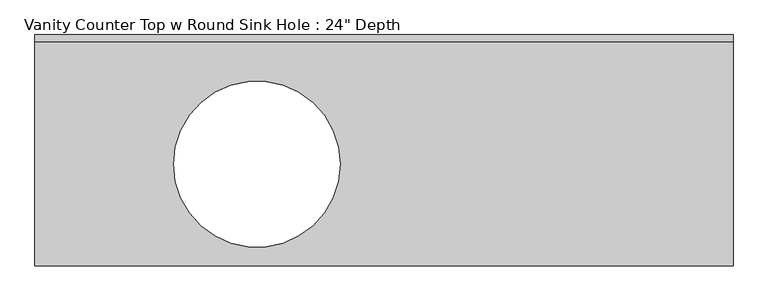
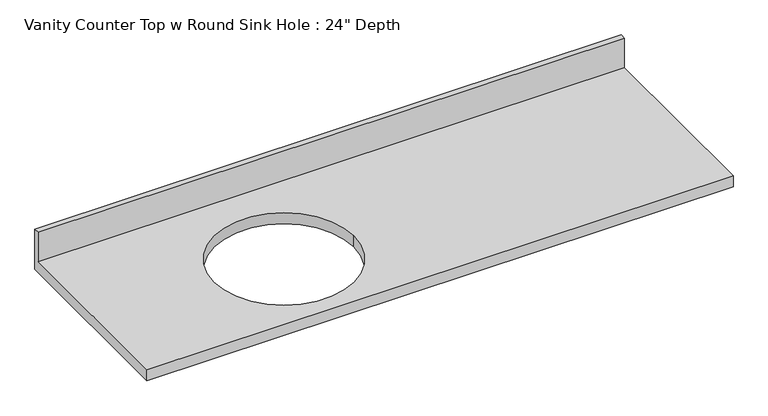
"""IFC4 building model written with IfcOpenShell, lengths in millimetres: furniture geometry."""

import ifcopenshell
import ifcopenshell.guid

model = None  # the IFC model being written
_history = None  # IfcOwnerHistory: only IFC2X3 demands one
_inside = {}  # id of a spatial element -> (the spatial element, [elements in it])
_under = {}  # id of a project, library or spatial element -> (it, [spatial elements below it])
_declared = {}  # id of a project -> (the project, [libraries it declares])
_typed = {}  # id of a type object -> (the type object, [elements of that type])
_made_of = {}  # id of a material, layer set ... -> (it, [elements and type objects made of it])


def new_model(schema):
    """Start an empty IFC model of exactly this schema.

    Asked for "IFC4X3", IfcOpenShell would pick the latest addendum, in which some entities
    have other attributes; the version numbers below select the first issue.
    IFC2X3 requires an IfcOwnerHistory on every rooted entity: one is made here for all.
    """
    global model, _history
    if schema == "IFC4X3":
        model = ifcopenshell.file(schema_version=(4, 3, 0, 0))
    else:
        model = ifcopenshell.file(schema=schema)
    _inside.clear()
    _under.clear()
    _declared.clear()
    _typed.clear()
    _made_of.clear()
    _history = None
    if model.schema == "IFC2X3":
        org = make("IfcOrganization", Name="unknown")
        user = make(
            "IfcPersonAndOrganization",
            ThePerson=make("IfcPerson", FamilyName="unknown"),
            TheOrganization=org,
        )
        app = make(
            "IfcApplication",
            ApplicationDeveloper=org,
            Version="unknown",
            ApplicationFullName="unknown",
            ApplicationIdentifier="unknown",
        )
        _history = make(
            "IfcOwnerHistory",
            OwningUser=user,
            OwningApplication=app,
            ChangeAction="ADDED",
            CreationDate=0,
        )
    return model


def make(cls, **values):
    """One entity of the class cls with the attributes given. An attribute that is None is left unset."""
    return model.create_entity(
        cls, **{name: value for name, value in values.items() if value is not None}
    )


def rooted(cls, **values):
    """An entity with a GlobalId (a new one), such as an element, a storey or a relation."""
    return make(cls, GlobalId=ifcopenshell.guid.new(), OwnerHistory=_history, **values)


def si_unit(unit_type, name, prefix=None):
    """IfcSIUnit, for example si_unit("LENGTHUNIT", "METRE", prefix="MILLI")."""
    return make("IfcSIUnit", UnitType=unit_type, Prefix=prefix, Name=name)


def assignment(units):
    """IfcUnitAssignment: the units of a project."""
    return None if units is None else make("IfcUnitAssignment", Units=units)


def point(xyz):
    """IfcCartesianPoint."""
    return None if xyz is None else make("IfcCartesianPoint", Coordinates=xyz)


def direction(xyz):
    """IfcDirection."""
    return None if xyz is None else make("IfcDirection", DirectionRatios=xyz)


def frame(location, z_axis=None, x_axis=None):
    """IfcAxis2Placement3D, a coordinate frame: its origin and axes. An axis left out is left unset."""
    return make(
        "IfcAxis2Placement3D",
        Location=point(location),
        Axis=direction(z_axis),
        RefDirection=direction(x_axis),
    )


def origin():
    """The frame at (0, 0, 0) with its axes left unset."""
    return frame((0.0, 0.0, 0.0))


def place(relative_to, where):
    """IfcLocalPlacement: puts the frame where relative to a parent placement (None: the world)."""
    return make(
        "IfcLocalPlacement", PlacementRelTo=relative_to, RelativePlacement=where
    )


def context(
    kind, dimensions, precision=None, world=None, true_north=None, identifier=None
):
    """IfcGeometricRepresentationContext, for example the 3D "Model" context."""
    return make(
        "IfcGeometricRepresentationContext",
        ContextIdentifier=identifier,
        ContextType=kind,
        CoordinateSpaceDimension=dimensions,
        Precision=precision,
        WorldCoordinateSystem=world,
        TrueNorth=true_north,
    )


def project(units=None, contexts=None):
    """IfcProject with its units and contexts."""
    return rooted(
        "IfcProject",
        Name="project",
        RepresentationContexts=contexts,
        UnitsInContext=assignment(units),
    )


def spatial(cls, under=None, at=None, **own):
    """A site, building, storey or space (cls), placed at a placement, below another one or the project."""
    s = rooted(cls, ObjectPlacement=at, **own)
    if under is not None:
        _under.setdefault(under.id(), (under, []))[1].append(s)
    return s


def polyline(points):
    """IfcPolyline through the points."""
    return make("IfcPolyline", Points=[point(p) for p in points])


def circle_curve(where, radius):
    """IfcCircle in the frame where."""
    return make("IfcCircle", Position=where, Radius=radius)


def shape(context_of_items, identifier, shape_type, items):
    """IfcShapeRepresentation: the items that make up one representation, for example the "Body"."""
    return make(
        "IfcShapeRepresentation",
        ContextOfItems=context_of_items,
        RepresentationIdentifier=identifier,
        RepresentationType=shape_type,
        Items=items,
    )


def source(mapping_origin, context_of_items, identifier, shape_type, items):
    """IfcRepresentationMap: a shape defined once, which mapped items show again and again."""
    return make(
        "IfcRepresentationMap",
        MappingOrigin=mapping_origin,
        MappedRepresentation=shape(context_of_items, identifier, shape_type, items),
    )


def transform(
    local_origin,
    x_axis=None,
    y_axis=None,
    z_axis=None,
    scale=None,
    scale2=None,
    scale3=None,
    uniform=True,
):
    """IfcCartesianTransformationOperator3D, or its non-uniform kind. x_axis, y_axis, z_axis: its Axis1, 2, 3."""
    if uniform:
        return make(
            "IfcCartesianTransformationOperator3D",
            Axis1=direction(x_axis),
            Axis2=direction(y_axis),
            LocalOrigin=point(local_origin),
            Scale=scale,
            Axis3=direction(z_axis),
        )
    return make(
        "IfcCartesianTransformationOperator3DnonUniform",
        Axis1=direction(x_axis),
        Axis2=direction(y_axis),
        LocalOrigin=point(local_origin),
        Scale=scale,
        Axis3=direction(z_axis),
        Scale2=scale2,
        Scale3=scale3,
    )


def mapped(mapping_source, mapping_target):
    """IfcMappedItem: shows the shape of a source again, moved by a transform."""
    return make(
        "IfcMappedItem", MappingSource=mapping_source, MappingTarget=mapping_target
    )


def made_of(thing, what):
    """Note that an element or type object is made of a material, layer set ...; save() writes the relation."""
    if what is not None:
        _made_of.setdefault(what.id(), (what, []))[1].append(thing)
    return thing


def element(
    cls,
    number,
    at=None,
    inside=None,
    cuts=None,
    type_object=None,
    material=None,
    context=None,
    identifier="Body",
    shape_type=None,
    held_by="IfcProductDefinitionShape",
    body=None,
    shapes=None,
    **own,
):
    """One element of the class cls, such as IfcWall. Its Tag is "e" and its number.

    at: its placement. inside: the storey or other place that contains it. cuts: it is an
    opening in that element (IfcRelVoidsElement). A single representation is given by context,
    identifier, shape_type and body (its items); several are given by shapes. held_by: the class
    of the entity that holds the representations. save() writes the other relations.
    """
    e = rooted(cls, Tag="e%d" % number, ObjectPlacement=at, **own)
    if body is not None:
        shapes = [shape(context, identifier, shape_type, body)]
    if shapes is not None:
        e.Representation = make(held_by, Representations=shapes)
    if inside is not None:
        _inside.setdefault(inside.id(), (inside, []))[1].append(e)
    if cuts is not None:
        rooted(
            "IfcRelVoidsElement", RelatingBuildingElement=cuts, RelatedOpeningElement=e
        )
    if type_object is not None:
        _typed.setdefault(type_object.id(), (type_object, []))[1].append(e)
    return made_of(e, material)


def aggregate(whole, parts):
    """IfcRelAggregates: a whole, such as a stair, and the parts it consists of."""
    return rooted("IfcRelAggregates", RelatingObject=whole, RelatedObjects=parts)


def save(model, path):
    """Write the relations noted so far, then the file.

    IfcRelAggregates (storeys below a building ...), IfcRelContainedInSpatialStructure (elements
    in a storey), IfcRelDefinesByType, IfcRelAssociatesMaterial and IfcRelDeclares: one each for
    every whole, place, type object, material and project.
    """
    for whole, parts in _under.values():
        aggregate(whole, parts)
    for where, things in _inside.values():
        rooted(
            "IfcRelContainedInSpatialStructure",
            RelatedElements=things,
            RelatingStructure=where,
        )
    for kind, things in _typed.values():
        rooted("IfcRelDefinesByType", RelatedObjects=things, RelatingType=kind)
    for what, things in _made_of.values():
        rooted("IfcRelAssociatesMaterial", RelatedObjects=things, RelatingMaterial=what)
    for by, libraries in _declared.values():
        rooted("IfcRelDeclares", RelatingContext=by, RelatedDefinitions=libraries)
    model.write(path)


def plane_surface(at):
    """IfcPlane: the flat surface through the origin of the frame at, square to its z axis."""
    return make("IfcPlane", Position=at)


def revolved_surface(curve, axis_point, axis_direction):
    """IfcSurfaceOfRevolution: the curve turned about the line through axis_point along axis_direction."""
    return make(
        "IfcSurfaceOfRevolution",
        SweptCurve=make("IfcArbitraryOpenProfileDef", ProfileType="CURVE", Curve=curve),
        AxisPosition=make("IfcAxis1Placement", Location=point(axis_point), Axis=direction(axis_direction)),
    )


def advanced_brep(points, edges, surfaces, faces):
    """IfcAdvancedBrep: a solid bounded by faces that lie on surfaces and meet in shared edges.

    An edge is (start, end): straight between two places in points (the first is 0);
    or (start, end, curve); or (start, end, curve, False) where it runs against its curve.
    A face is (place in surfaces, loops), or (place, loops, False) where it looks against
    its surface's normal. A loop lists edges by number (the first is 1), with a minus sign
    where the edge is run from its end to its start. The first loop is the outer one.
    """
    corners = [point(p) for p in points]
    vertices = [make("IfcVertexPoint", VertexGeometry=c) for c in corners]
    made = []
    for start, end, *more in edges:
        made.append(
            make(
                "IfcEdgeCurve",
                EdgeStart=vertices[start],
                EdgeEnd=vertices[end],
                EdgeGeometry=more[0] if more else make("IfcPolyline", Points=[corners[start], corners[end]]),
                SameSense=more[1] if len(more) > 1 else True,
            )
        )
    hull = []
    for where, loops, *sense in faces:
        bounds = []
        for j, loop in enumerate(loops):
            ring = [make("IfcOrientedEdge", EdgeElement=made[abs(k) - 1], Orientation=k > 0) for k in loop]
            bounds.append(
                make(
                    "IfcFaceOuterBound" if j == 0 else "IfcFaceBound",
                    Bound=make("IfcEdgeLoop", EdgeList=ring),
                    Orientation=True,
                )
            )
        hull.append(make("IfcAdvancedFace", Bounds=bounds, FaceSurface=surfaces[where], SameSense=sense[0] if sense else True))
    return make("IfcAdvancedBrep", Outer=make("IfcClosedShell", CfsFaces=hull))


def furniture_79ec22a3(model_context):
    return source(origin(), model_context, "Body", "AdvancedBrep", [
        advanced_brep(
        [(-1327.4622951, -635.0, 787.4), (590.2377049, -635.0, 787.4), (590.2377049, -19.05, 787.4), (-1327.4622951, -19.05, 787.4), (-489.2622951, -355.6, 787.4), (-946.4622951, -355.6, 787.4), (590.2377049, 0.0, 749.3), (590.2377049, -635.0, 749.3), (-1327.4622951, -635.0, 749.3), (-1327.4622951, 0.0, 749.3), (-946.4622951, -355.6, 749.3), (-489.2622951, -355.6, 749.3), (-1327.4622951, 0.0, 889.0), (590.2377049, 0.0, 889.0), (-1327.4622951, -19.05, 889.0), (590.2377049, -19.05, 889.0)],
        [
            (0, 1),
            (1, 2),
            (2, 3),
            (3, 0),
            (4, 5, circle_curve(frame((-717.8622951, -355.6, 787.4), z_axis=(0.0, 0.0, -1.0), x_axis=(1.0, 0.0, 0.0)), 228.6)),
            (5, 4, circle_curve(frame((-717.8622951, -355.6, 787.4), z_axis=(0.0, 0.0, -1.0), x_axis=(1.0, 0.0, 0.0)), 228.6)),
            (6, 7),
            (7, 8),
            (8, 9),
            (9, 6),
            (10, 11, circle_curve(frame((-717.8622951, -355.6, 749.3), z_axis=(0.0, 0.0, 1.0), x_axis=(1.0, 0.0, 0.0)), 228.6)),
            (11, 10, circle_curve(frame((-717.8622951, -355.6, 749.3), z_axis=(0.0, 0.0, 1.0), x_axis=(1.0, 0.0, 0.0)), 228.6)),
            (9, 12),
            (12, 13),
            (13, 6),
            (8, 0),
            (3, 14),
            (14, 12),
            (7, 1),
            (13, 15),
            (15, 2),
            (14, 15),
            (4, 11),
            (10, 5),
        ],
        [
            plane_surface(frame((-1327.4622951, 0.0, 787.4), z_axis=(0.0, 0.0, 1.0), x_axis=(-1.0, 0.0, 0.0))),
            plane_surface(frame((-1327.4622951, 0.0, 749.3), z_axis=(0.0, 0.0, -1.0), x_axis=(1.0, 0.0, 0.0))),
            plane_surface(frame((590.2377049, 0.0, 787.4), z_axis=(0.0, 1.0, 0.0), x_axis=(0.0, 0.0, -1.0))),
            plane_surface(frame((-1327.4622951, 0.0, 787.4), z_axis=(-1.0, 0.0, 0.0), x_axis=(0.0, 0.0, -1.0))),
            plane_surface(frame((-1327.4622951, -635.0, 787.4), z_axis=(0.0, -1.0, 0.0), x_axis=(0.0, 0.0, -1.0))),
            plane_surface(frame((590.2377049, -635.0, 787.4), z_axis=(1.0, 0.0, 0.0), x_axis=(0.0, 0.0, -1.0))),
            plane_surface(frame((-1327.4622951, 0.0, 889.0), z_axis=(0.0, 0.0, 1.0), x_axis=(0.0, -1.0, 0.0))),
            plane_surface(frame((-1327.4622951, -19.05, 889.0), z_axis=(0.0, -1.0, 0.0), x_axis=(0.0, 0.0, -1.0))),
            revolved_surface(polyline([(-489.26229509999996, -355.6, 787.4), (-489.26229509999996, -355.6, 749.3)]), (-717.8622951, -355.6, 749.3), (0.0, 0.0, 1.0)),
        ],
        [
            (0, [[1, 2, 3, 4], [5, 6]]),
            (1, [[7, 8, 9, 10], [11, 12]]),
            (2, [[-10, 13, 14, 15]]),
            (3, [[-9, 16, -4, 17, 18, -13]]),
            (4, [[-1, -16, -8, 19]]),
            (5, [[-7, -15, 20, 21, -2, -19]]),
            (6, [[-18, 22, -20, -14]]),
            (7, [[-22, -17, -3, -21]]),
            (8, [[23, -11, 24, -5]]),
            (8, [[-23, -6, -24, -12]]),
        ],
    ),
    ])


if __name__ == "__main__":
    model = new_model("IFC4")
    model_context = context("Model", 3, world=origin())
    ifc_project = project(units=[si_unit("LENGTHUNIT", "METRE", prefix="MILLI")], contexts=[model_context])
    site = spatial("IfcSite", under=ifc_project)
    building = spatial("IfcBuilding", under=site)
    placement = place(None, origin())
    furniture_shape = furniture_79ec22a3(model_context)
    element("IfcFurniture", 1, ObjectType="Vanity Counter Top w Round Sink Hole : 24\" Depth", at=placement, inside=building, context=model_context, shape_type="MappedRepresentation", body=[
        mapped(furniture_shape, transform((0.0, 0.0, 0.0), x_axis=(1.0, 0.0, 0.0), y_axis=(0.0, 1.0, 0.0), z_axis=(0.0, 0.0, 1.0))),
    ])
    save(model, "model.ifc")

# Revit data of these elements
# Type "Vanity Counter Top w Round Sink Hole : 24\" Depth"
#   Assembly Code = "C1030400"
#   Counter Thickness = 0' - 1 1/2"
#   Depth = 2' - 1"
#   Height = 2' - 7"
#   Length [instance default] = 4' - 0"
#   Sink Location [instance default] = 2' - 0"
#   Sink Location To Wall [instance default] = 0' - 4"
#   Sink Opening Width [instance default] = 1' - 5"
#   Counter Top Material = Laminate, Blue, Matte
#   Default Elevation = 0
# Element 1 (IfcFurniture, "Vanity Counter Top w Round Sink Hole : 24\" Depth")
#   Length = 6' - 3 1/2"
#   Sink Location To Wall = 0' - 5 1/2"
#   Materials on its faces: "Laminate, Blue, Matte"
# Materials
#   "Laminate, Blue, Matte": class "Plastic", colour RGB 85 101 155, transparency 0, Description = "Plastic Laminate - Blue, Matte", Cost = 0
